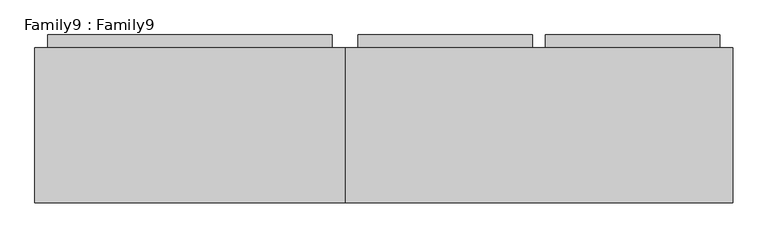
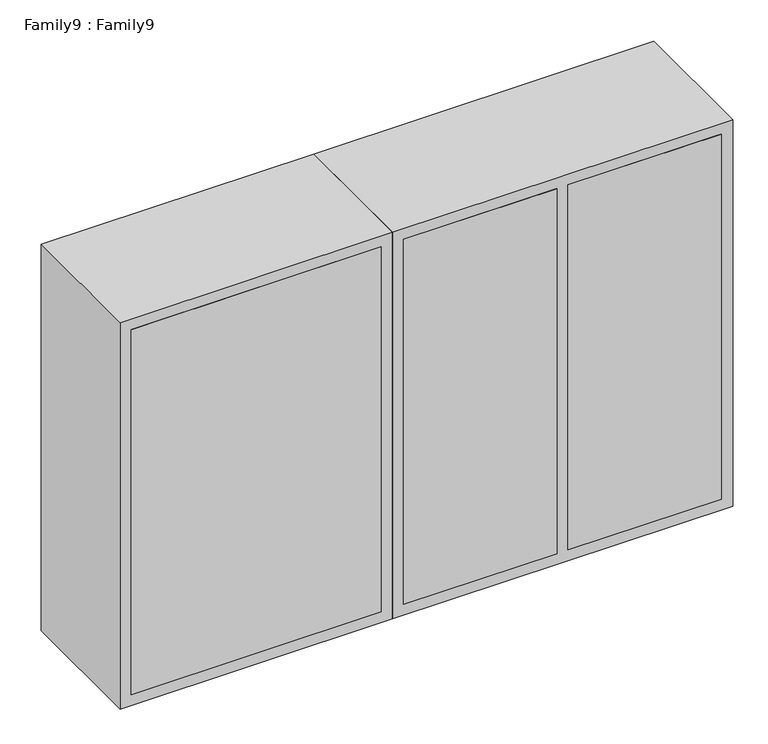
"""IFC4 building model written with IfcOpenShell, lengths in millimetres: proxy geometry, Family9 : Family9."""

from ifc_helpers import new_model, si_unit, frame, origin, place, context, project, spatial, polyline, outline, extrude, source, transform, mapped, element, save


def family9_family9_df6b3b5b(model_context):
    return source(origin(), model_context, "Body", "SweptSolid", [
        extrude(outline(polyline([(-965.2, 381.0), (-406.4, 381.0), (-406.4, 50.8), (-965.2, 50.8), (-965.2, 381.0)])), frame((0.0, 0.0, 1209.1599575), z_axis=(0.0, 0.0, 1.0), x_axis=(1.0, 0.0, 0.0)), (0.0, 0.0, 1.0), 863.6),
        extrude(outline(polyline([(-990.6, 355.6), (-381.0, 355.6), (-381.0, 50.8), (-990.6, 50.8), (-990.6, 355.6)])), frame((0.0, 0.0, 1183.7599575), z_axis=(0.0, 0.0, 1.0), x_axis=(1.0, 0.0, 0.0)), (0.0, 0.0, 1.0), 914.4),
        extrude(outline(polyline([(12.7, 381.0), (355.6, 381.0), (355.6, 50.8), (12.7, 50.8), (12.7, 381.0)])), frame((0.0, 0.0, 1209.1599575), z_axis=(0.0, 0.0, 1.0), x_axis=(1.0, 0.0, 0.0)), (0.0, 0.0, 1.0), 863.6),
        extrude(outline(polyline([(-355.6, 381.0), (-12.7, 381.0), (-12.7, 50.8), (-355.6, 50.8), (-355.6, 381.0)])), frame((0.0, 0.0, 1209.1599575), z_axis=(0.0, 0.0, 1.0), x_axis=(1.0, 0.0, 0.0)), (0.0, 0.0, 1.0), 863.6),
        extrude(outline(polyline([(-381.0, 355.6), (381.0, 355.6), (381.0, 50.8), (-381.0, 50.8), (-381.0, 355.6)])), frame((0.0, 0.0, 1183.7599575), z_axis=(0.0, 0.0, 1.0), x_axis=(1.0, 0.0, 0.0)), (0.0, 0.0, 1.0), 914.4),
    ])


if __name__ == "__main__":
    model = new_model("IFC4")
    model_context = context("Model", 3, world=origin())
    ifc_project = project(units=[si_unit("LENGTHUNIT", "METRE", prefix="MILLI")], contexts=[model_context])
    site = spatial("IfcSite", under=ifc_project)
    building = spatial("IfcBuilding", under=site)
    placement = place(None, origin())
    family9_family9_shape = family9_family9_df6b3b5b(model_context)
    element("IfcBuildingElementProxy", 1, Name="Family9 : Family9", ObjectType="Family9 : Family9", at=placement, inside=building, context=model_context, shape_type="MappedRepresentation", body=[
        mapped(family9_family9_shape, transform((0.0, 0.0, 0.0), x_axis=(1.0, 0.0, 0.0), y_axis=(0.0, 1.0, 0.0), z_axis=(0.0, 0.0, 1.0))),
    ])
    save(model, "model.ifc")

# Revit data of these elements
# Type "Family9 : Family9"
#   drawer depth = 1' - 1"
#   cabinet depth = 1' - 0"
#   Default Elevation = 0
